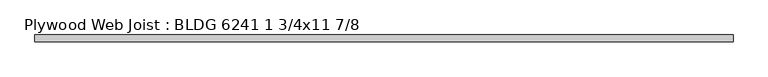
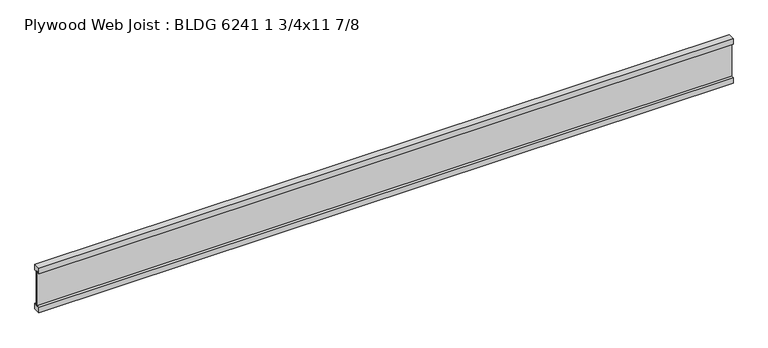
"""IFC4 building model written with IfcOpenShell, lengths in millimetres: beam geometry, Plywood Web Joist : BLDG 6241 1 3/4x11 7/8."""

from ifc_helpers import new_model, si_unit, frame, origin, place, context, project, spatial, polyline, outline, extrude, source, transform, mapped, element, save


def plywood_web_joist_bldg_6241_1_3_4x11_7_8_a42695ab(model_context):
    return source(origin(), model_context, "Body", "SweptSolid", [
        extrude(outline(polyline([(-22.225, 150.8125), (22.225, 150.8125), (22.225, 112.7125), (4.7625, 112.7125), (4.7625, 119.0625), (-4.7625, 119.0625), (-4.7625, 112.7125), (-22.225, 112.7125), (-22.225, 150.8125)])), frame((-2232.025, 0.0, 0.0), z_axis=(1.0, 0.0, 0.0), x_axis=(0.0, 1.0, 0.0)), (0.0, 0.0, 1.0), 4464.05),
        extrude(outline(polyline([(22.225, -112.7125), (22.225, -150.8125), (-22.225, -150.8125), (-22.225, -112.7125), (-4.7625, -112.7125), (-4.7625, -118.3285374), (4.7625, -118.3285374), (4.7625, -112.7125), (22.225, -112.7125)])), frame((-2232.025, 0.0, 0.0), z_axis=(1.0, 0.0, 0.0), x_axis=(0.0, 1.0, 0.0)), (0.0, 0.0, 1.0), 4464.05),
        extrude(outline(polyline([(2232.025, 4.7625), (2232.025, -4.7625), (-2232.025, -4.7625), (-2232.025, 4.7625), (2232.025, 4.7625)])), frame((0.0, 0.0, -118.3285374), z_axis=(0.0, 0.0, 1.0), x_axis=(1.0, 0.0, 0.0)), (0.0, 0.0, 1.0), 237.3910374),
    ])


if __name__ == "__main__":
    model = new_model("IFC4")
    model_context = context("Model", 3, world=origin())
    ifc_project = project(units=[si_unit("LENGTHUNIT", "METRE", prefix="MILLI")], contexts=[model_context])
    site = spatial("IfcSite", under=ifc_project)
    building = spatial("IfcBuilding", under=site)
    placement = place(None, origin())
    plywood_web_joist_bldg_6241_1_3_4x11_7_8_shape = plywood_web_joist_bldg_6241_1_3_4x11_7_8_a42695ab(model_context)
    element("IfcBeam", 1, ObjectType="Plywood Web Joist : BLDG 6241 1 3/4x11 7/8", at=placement, inside=building, context=model_context, shape_type="MappedRepresentation", body=[
        mapped(plywood_web_joist_bldg_6241_1_3_4x11_7_8_shape, transform((0.0, 0.0, 0.0), x_axis=(1.0, 0.0, 0.0), y_axis=(0.0, 1.0, 0.0), z_axis=(0.0, 0.0, 1.0))),
    ])
    save(model, "model.ifc")

# Revit data of these elements
# Type "Plywood Web Joist : BLDG 6241 1 3/4x11 7/8"
#   Assembly Code = "B10"
#   Length [instance default] = 5' - 0"
#   b = 0' - 1 3/4"
#   d = 0' - 11 7/8"
#   Structural Material [instance default] = Softwood, Lumber
# Element 1 (IfcBeam, "Plywood Web Joist : BLDG 6241 1 3/4x11 7/8")
#   Materials on its faces: "Softwood, Lumber"
# Materials
#   "Softwood, Lumber": class "Wood", colour RGB 223 192 134, transparency 0, Description = "Pinus Echinata", Cost = 0
